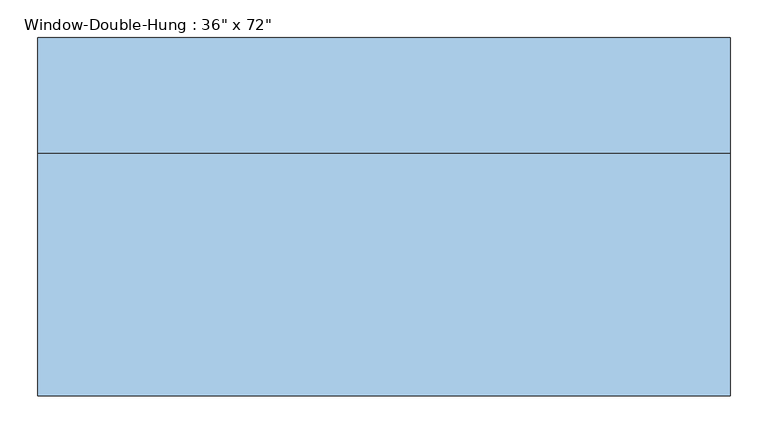
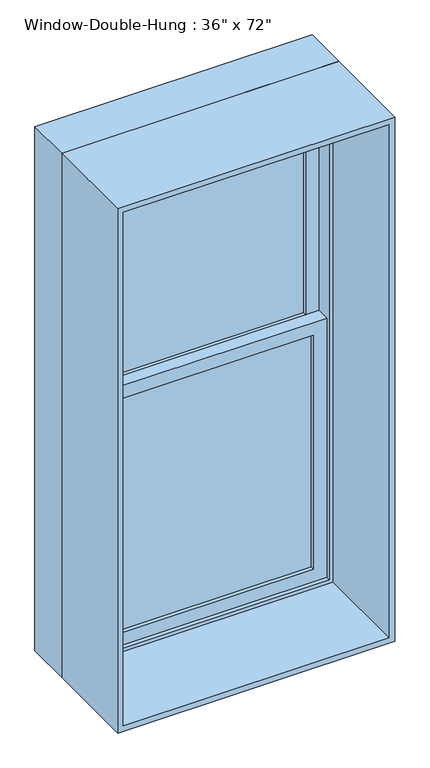
"""IFC4 building model written with IfcOpenShell, lengths in millimetres: window geometry."""

from ifc_helpers import new_model, si_unit, frame, origin, place, context, project, spatial, polyline, outline, extrude, source, transform, mapped, element, save


def window_94ba0d48(model_context):
    return source(origin(), model_context, "Body", "SweptSolid", [
        extrude(outline(polyline([(381.0, 138.1125), (381.0, 131.7625), (-381.0, 131.7625), (-381.0, 138.1125), (381.0, 138.1125)])), frame((0.0, 0.0, 990.6), z_axis=(0.0, 0.0, 1.0), x_axis=(1.0, 0.0, 0.0)), (0.0, 0.0, 1.0), 815.975),
        extrude(outline(polyline([(-381.0, 125.4125), (381.0, 125.4125), (381.0, 119.0625), (-381.0, 119.0625), (-381.0, 125.4125)])), frame((0.0, 0.0, 990.6), z_axis=(0.0, 0.0, 1.0), x_axis=(1.0, 0.0, 0.0)), (0.0, 0.0, 1.0), 815.975),
        extrude(outline(polyline([(381.0, 182.5625), (381.0, 176.2125), (-381.0, 176.2125), (-381.0, 182.5625), (381.0, 182.5625)])), frame((0.0, 0.0, 1851.025), z_axis=(0.0, 0.0, 1.0), x_axis=(1.0, 0.0, 0.0)), (0.0, 0.0, 1.0), 815.975),
        extrude(outline(polyline([(-381.0, 169.8625), (381.0, 169.8625), (381.0, 163.5125), (-381.0, 163.5125), (-381.0, 169.8625)])), frame((0.0, 0.0, 1851.025), z_axis=(0.0, 0.0, 1.0), x_axis=(1.0, 0.0, 0.0)), (0.0, 0.0, 1.0), 815.975),
        extrude(outline(polyline([(1851.025, -425.45), (946.15, -425.45), (946.15, 425.45), (1851.025, 425.45), (1851.025, -425.45)]), holes=[polyline([(1806.575, 381.0), (990.6, 381.0), (990.6, -381.0), (1806.575, -381.0), (1806.575, 381.0)])]), frame((0.0, 106.3625, 0.0), z_axis=(0.0, 1.0, 0.0), x_axis=(0.0, 0.0, 1.0)), (0.0, 0.0, 1.0), 44.45),
        extrude(outline(polyline([(2711.45, -425.45), (1806.575, -425.45), (1806.575, 425.45), (2711.45, 425.45), (2711.45, -425.45)]), holes=[polyline([(2667.0, 381.0), (1851.025, 381.0), (1851.025, -381.0), (2667.0, -381.0), (2667.0, 381.0)])]), frame((0.0, 150.8125, 0.0), z_axis=(0.0, 1.0, 0.0), x_axis=(0.0, 0.0, 1.0)), (0.0, 0.0, 1.0), 44.45),
        extrude(outline(polyline([(2743.2, -457.2), (914.4, -457.2), (914.4, 457.2), (2743.2, 457.2), (2743.2, -457.2)]), holes=[polyline([(2711.45, 425.45), (946.15, 425.45), (946.15, -425.45), (2711.45, -425.45), (2711.45, 425.45)])]), frame((0.0, 93.6625, 0.0), z_axis=(0.0, 1.0, 0.0), x_axis=(0.0, 0.0, 1.0)), (0.0, 0.0, 1.0), 152.4),
        extrude(outline(polyline([(2743.2, 457.2), (2743.2, -457.2), (914.4, -457.2), (914.4, 457.2), (2743.2, 457.2)]), holes=[polyline([(2724.15, 438.15), (933.45, 438.15), (933.45, -438.15), (2724.15, -438.15), (2724.15, 438.15)])]), frame((0.0, -227.0125, 0.0), z_axis=(0.0, 1.0, 0.0), x_axis=(0.0, 0.0, 1.0)), (0.0, 0.0, 1.0), 320.675),
    ])


if __name__ == "__main__":
    model = new_model("IFC4")
    model_context = context("Model", 3, world=origin())
    ifc_project = project(units=[si_unit("LENGTHUNIT", "METRE", prefix="MILLI")], contexts=[model_context])
    site = spatial("IfcSite", under=ifc_project)
    building = spatial("IfcBuilding", under=site)
    placement = place(None, origin())
    window_shape = window_94ba0d48(model_context)
    element("IfcWindow", 1, ObjectType="Window-Double-Hung : 36\" x 72\"", at=placement, inside=building, context=model_context, shape_type="MappedRepresentation", body=[
        mapped(window_shape, transform((0.0, 0.0, 0.0), x_axis=(1.0, 0.0, 0.0), y_axis=(0.0, 1.0, 0.0), z_axis=(0.0, 0.0, 1.0))),
    ])
    save(model, "model.ifc")

# Revit data of these elements
# Type "Window-Double-Hung : 36\" x 72\""
#   Type Mark = "22"
#   Fire Rating = "0.5h"
#   Construction Type Id = "DG-DR"
#   Assembly Code = "B2020100"
#   Analytic Construction = "Double glazing - domestic"
#   Wall Thickness [instance default] = 0' - 6"
#   Visual Light Transmittance = 0.81
#   Thermal Resistance (R) = 1.8146 (h·ft²·°F)/BTU
#   Solar Heat Gain Coefficient = 0.76
#   Rough Width = 3' - 0 1/2"
#   Rough Height = 6' - 0 1/2"
#   Muntin Width = 2' - 6"
#   Muntin Height = 2' - 8 1/8"
#   Interior Wall Closure [instance default] = 0' - 1 1/2"
#   Heat Transfer Coefficient (U) = 0.5511 BTU/(h·ft²·°F)
#   Frame Extension [instance default] = 0' - 2"
#   Exterior Wall Closure [instance default] = 0' - 0 1/2"
#   Extension Jamb [instance default] = 0' - 0 3/4"
#   Height = 6' - 0"
#   Width = 3' - 0"
#   Window Inset [instance default] = 0' - 0 3/4"
#   Top Muntin Visibility = yes
#   Interior Trim Visibility [instance default] = yes
#   Indicator Visibility [instance default] = yes
#   Exterior Trim Visibility [instance default] = yes
#   Extension Jamb Visibility [instance default] = yes
#   Define Thermal Properties by = 1
#   Bottom Muntin Visibility = yes
#   Muntin Pattern = Muntin Pattern_2x2 : Muntin Pattern_2x2
#   Interior Trim Material = Wood - Stained
#   Interior Trim = Trim-Window-Interior-Flat : Picture Frame
#   Interior Frame Material = Wood - Stained
#   Glass Panel Material = Glass
#   Exterior Trim Material = Clad - White
#   Exterior Trim = Trim-Window-Exterior-Flat : with Sill
#   Exterior Frame Material = Clad - White
#   Wall Closure = (empty or 0)
# Element 1 (IfcWindow, "Window-Double-Hung : 36\" x 72\"")
#   Wall Thickness = 1' - 5 7/8"
#   Extension Jamb = 1' - 0 5/8"
#   Materials on its faces: "Wood - Stained", "Glass", "Clad - White"
# Materials
#   "Wood - Stained": class "Wood", colour RGB 224 178 126, transparency 0, Cost = 0
#   "Glass": class "Unassigned", colour RGB 0 128 192, transparency 0.75, Description = "Glass"
#   "Clad - White": class "Wood", colour RGB 242 242 238, transparency 0, Cost = 0
